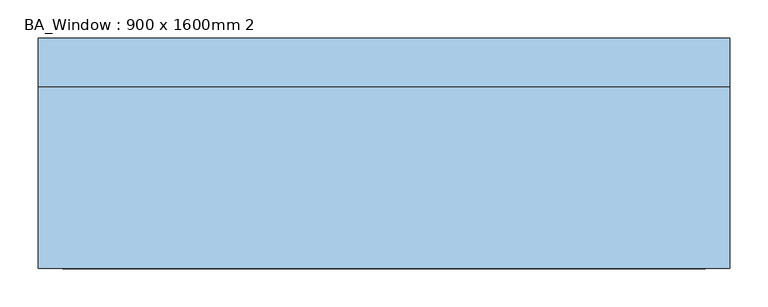
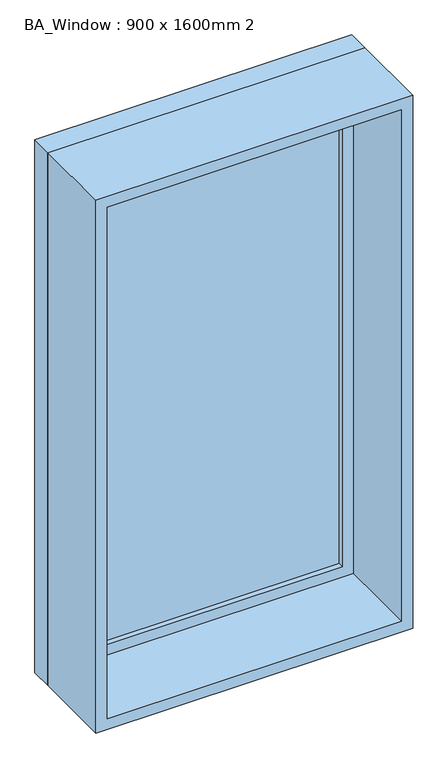
"""IFC4 building model written with IfcOpenShell, lengths in millimetres: window geometry, BA_Window : 900 x 1600mm 2."""

from ifc_helpers import new_model, si_unit, frame, origin, place, context, project, spatial, polyline, outline, extrude, source, transform, mapped, element, save


def ba_window_900_x_1600mm_2_0de2e490(model_context):
    return source(origin(), model_context, "Body", "SweptSolid", [
        extrude(outline(polyline([(-387.0, 128.0), (387.0, 128.0), (387.0, 116.0), (-387.0, 116.0), (-387.0, 128.0)])), frame((0.0, 0.0, 978.0), z_axis=(0.0, 0.0, 1.0), x_axis=(1.0, 0.0, 0.0)), (0.0, 0.0, 1.0), 1474.0),
        extrude(outline(polyline([(2496.0, -431.0), (934.0, -431.0), (934.0, 431.0), (2496.0, 431.0), (2496.0, -431.0)]), holes=[polyline([(2452.0, -387.0), (2452.0, 387.0), (978.0, 387.0), (978.0, -387.0), (2452.0, -387.0)])]), frame((0.0, 100.0, 0.0), z_axis=(0.0, 1.0, 0.0), x_axis=(0.0, 0.0, 1.0)), (0.0, 0.0, 1.0), 44.0),
        extrude(outline(polyline([(2515.0, -450.0), (915.0, -450.0), (915.0, 450.0), (2515.0, 450.0), (2515.0, -450.0)]), holes=[polyline([(2496.0, -431.0), (2496.0, 431.0), (934.0, 431.0), (934.0, -431.0), (2496.0, -431.0)])]), frame((0.0, 100.0, 0.0), z_axis=(0.0, 1.0, 0.0), x_axis=(0.0, 0.0, 1.0)), (0.0, 0.0, 1.0), 63.0),
        extrude(outline(polyline([(2515.0, -450.0), (915.0, -450.0), (915.0, 450.0), (2515.0, 450.0), (2515.0, -450.0)]), holes=[polyline([(2483.0, -418.0), (2483.0, 418.0), (947.0, 418.0), (947.0, -418.0), (2483.0, -418.0)])]), frame((0.0, -137.0, 0.0), z_axis=(0.0, 1.0, 0.0), x_axis=(0.0, 0.0, 1.0)), (0.0, 0.0, 1.0), 237.0),
    ])


if __name__ == "__main__":
    model = new_model("IFC4")
    model_context = context("Model", 3, world=origin())
    ifc_project = project(units=[si_unit("LENGTHUNIT", "METRE", prefix="MILLI")], contexts=[model_context])
    site = spatial("IfcSite", under=ifc_project)
    building = spatial("IfcBuilding", under=site)
    placement = place(None, origin())
    ba_window_900_x_1600mm_2_shape = ba_window_900_x_1600mm_2_0de2e490(model_context)
    element("IfcWindow", 1, ObjectType="BA_Window : 900 x 1600mm 2", at=placement, inside=building, context=model_context, shape_type="MappedRepresentation", body=[
        mapped(ba_window_900_x_1600mm_2_shape, transform((0.0, 0.0, 0.0), x_axis=(1.0, 0.0, 0.0), y_axis=(0.0, 1.0, 0.0), z_axis=(0.0, 0.0, 1.0))),
    ])
    save(model, "model.ifc")

# Revit data of these elements
# Project information
#   Project Issue Date = "Issue Date"
#   Project Status = "Project Status"
#   Client Name = "Owner"
#   Project Address = "Enter address here"
#   Project Name = "Project Name"
#   Project Number = "0001"
# Type "BA_Window : 900 x 1600mm 2"
#   Type Mark = "40"
#   Construction Type Id = "GSP4R"
#   Analytic Construction = "1/8 in Pilkington single glazing"
#   Visual Light Transmittance = 0.9
#   Thermal Resistance (R) = 0.271106 (m²·K)/W
#   Solar Heat Gain Coefficient = 0.78
#   Heat Transfer Coefficient (U) = 3.6886 W/(m²·K)
#   Height = 1600 mm
#   Default Sill Height = 915 mm
#   Width = 900 mm
#   Window Inset = 19 mm
#   Define Thermal Properties by = 1
#   Frame Exterior Material = Default
#   Frame Interior Material = Default
#   Glass Pane Material = Glass
#   Sash = Default
#   Wall Closure = (empty or 0)
# Element 1 (IfcWindow, "BA_Window : 900 x 1600mm 2")
#   Materials on its faces: "Default", "Glass"
# Materials
#   "Default": class "Generic", colour RGB 255 255 255, transparency 0, Cost = 0
#   "Glass": class "Glass", colour RGB 0 128 192, transparency 0.9, Description = "Soda Lime Glass", Cost = 0
